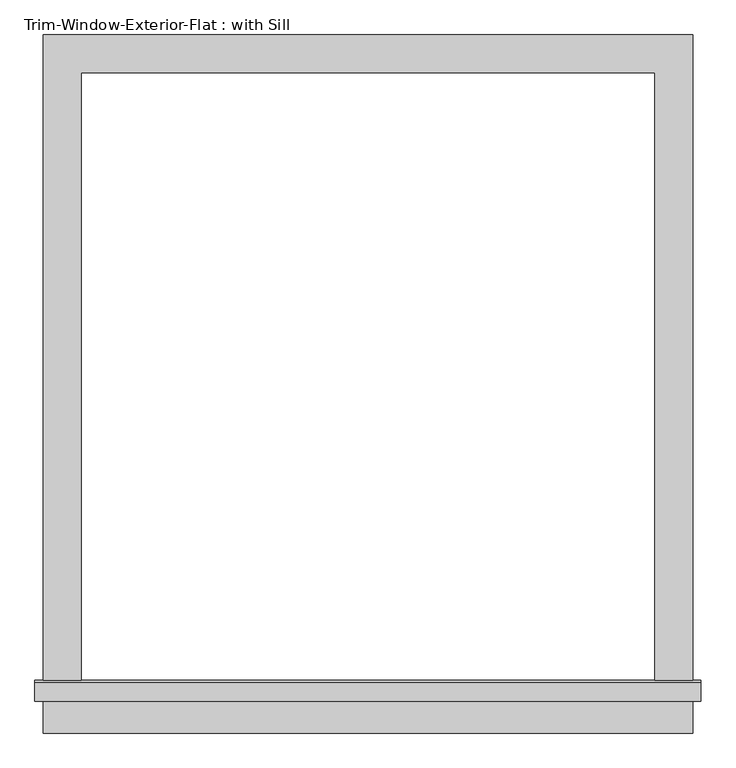
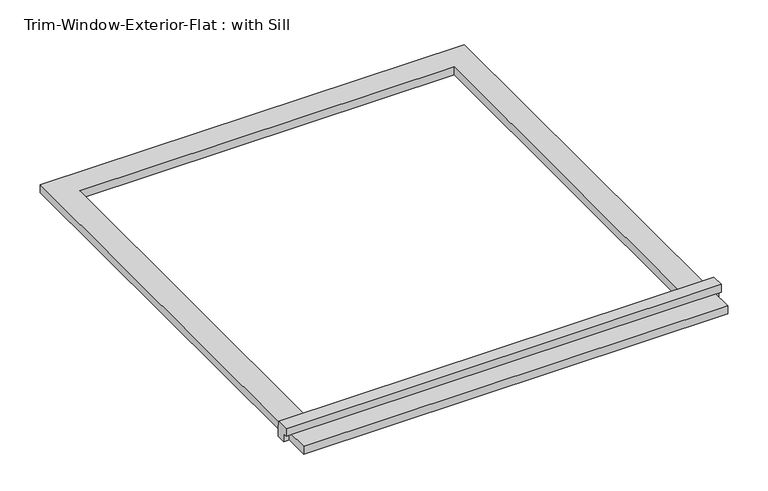
"""IFC4 building model written with IfcOpenShell, lengths in millimetres: proxy geometry, Trim-Window-Exterior-Flat : with Sill."""

import ifcopenshell
import ifcopenshell.guid

model = None  # the IFC model being written
_history = None  # IfcOwnerHistory: only IFC2X3 demands one
_inside = {}  # id of a spatial element -> (the spatial element, [elements in it])
_under = {}  # id of a project, library or spatial element -> (it, [spatial elements below it])
_declared = {}  # id of a project -> (the project, [libraries it declares])
_typed = {}  # id of a type object -> (the type object, [elements of that type])
_made_of = {}  # id of a material, layer set ... -> (it, [elements and type objects made of it])


def new_model(schema):
    """Start an empty IFC model of exactly this schema.

    Asked for "IFC4X3", IfcOpenShell would pick the latest addendum, in which some entities
    have other attributes; the version numbers below select the first issue.
    IFC2X3 requires an IfcOwnerHistory on every rooted entity: one is made here for all.
    """
    global model, _history
    if schema == "IFC4X3":
        model = ifcopenshell.file(schema_version=(4, 3, 0, 0))
    else:
        model = ifcopenshell.file(schema=schema)
    _inside.clear()
    _under.clear()
    _declared.clear()
    _typed.clear()
    _made_of.clear()
    _history = None
    if model.schema == "IFC2X3":
        org = make("IfcOrganization", Name="unknown")
        user = make(
            "IfcPersonAndOrganization",
            ThePerson=make("IfcPerson", FamilyName="unknown"),
            TheOrganization=org,
        )
        app = make(
            "IfcApplication",
            ApplicationDeveloper=org,
            Version="unknown",
            ApplicationFullName="unknown",
            ApplicationIdentifier="unknown",
        )
        _history = make(
            "IfcOwnerHistory",
            OwningUser=user,
            OwningApplication=app,
            ChangeAction="ADDED",
            CreationDate=0,
        )
    return model


def make(cls, **values):
    """One entity of the class cls with the attributes given. An attribute that is None is left unset."""
    return model.create_entity(
        cls, **{name: value for name, value in values.items() if value is not None}
    )


def rooted(cls, **values):
    """An entity with a GlobalId (a new one), such as an element, a storey or a relation."""
    return make(cls, GlobalId=ifcopenshell.guid.new(), OwnerHistory=_history, **values)


def si_unit(unit_type, name, prefix=None):
    """IfcSIUnit, for example si_unit("LENGTHUNIT", "METRE", prefix="MILLI")."""
    return make("IfcSIUnit", UnitType=unit_type, Prefix=prefix, Name=name)


def assignment(units):
    """IfcUnitAssignment: the units of a project."""
    return None if units is None else make("IfcUnitAssignment", Units=units)


def point(xyz):
    """IfcCartesianPoint."""
    return None if xyz is None else make("IfcCartesianPoint", Coordinates=xyz)


def direction(xyz):
    """IfcDirection."""
    return None if xyz is None else make("IfcDirection", DirectionRatios=xyz)


def frame(location, z_axis=None, x_axis=None):
    """IfcAxis2Placement3D, a coordinate frame: its origin and axes. An axis left out is left unset."""
    return make(
        "IfcAxis2Placement3D",
        Location=point(location),
        Axis=direction(z_axis),
        RefDirection=direction(x_axis),
    )


def origin():
    """The frame at (0, 0, 0) with its axes left unset."""
    return frame((0.0, 0.0, 0.0))


def origin_with_axes():
    """The frame at (0, 0, 0) with the z axis (0, 0, 1) and the x axis (1, 0, 0) written out."""
    return frame((0.0, 0.0, 0.0), z_axis=(0.0, 0.0, 1.0), x_axis=(1.0, 0.0, 0.0))


def place(relative_to, where):
    """IfcLocalPlacement: puts the frame where relative to a parent placement (None: the world)."""
    return make(
        "IfcLocalPlacement", PlacementRelTo=relative_to, RelativePlacement=where
    )


def context(
    kind, dimensions, precision=None, world=None, true_north=None, identifier=None
):
    """IfcGeometricRepresentationContext, for example the 3D "Model" context."""
    return make(
        "IfcGeometricRepresentationContext",
        ContextIdentifier=identifier,
        ContextType=kind,
        CoordinateSpaceDimension=dimensions,
        Precision=precision,
        WorldCoordinateSystem=world,
        TrueNorth=true_north,
    )


def project(units=None, contexts=None):
    """IfcProject with its units and contexts."""
    return rooted(
        "IfcProject",
        Name="project",
        RepresentationContexts=contexts,
        UnitsInContext=assignment(units),
    )


def spatial(cls, under=None, at=None, **own):
    """A site, building, storey or space (cls), placed at a placement, below another one or the project."""
    s = rooted(cls, ObjectPlacement=at, **own)
    if under is not None:
        _under.setdefault(under.id(), (under, []))[1].append(s)
    return s


def polyline(points):
    """IfcPolyline through the points."""
    return make("IfcPolyline", Points=[point(p) for p in points])


def outline(outer, holes=None, kind="AREA"):
    """IfcArbitraryClosedProfileDef: a profile drawn as a closed curve; with holes, ...WithVoids."""
    if holes is None:
        return make("IfcArbitraryClosedProfileDef", ProfileType=kind, OuterCurve=outer)
    return make(
        "IfcArbitraryProfileDefWithVoids",
        ProfileType=kind,
        OuterCurve=outer,
        InnerCurves=holes,
    )


def extrude(swept, where, along, depth):
    """IfcExtrudedAreaSolid: the profile swept, set in the frame where, extruded along a direction by depth."""
    return make(
        "IfcExtrudedAreaSolid",
        SweptArea=swept,
        Position=where,
        ExtrudedDirection=direction(along),
        Depth=depth,
    )


def shape(context_of_items, identifier, shape_type, items):
    """IfcShapeRepresentation: the items that make up one representation, for example the "Body"."""
    return make(
        "IfcShapeRepresentation",
        ContextOfItems=context_of_items,
        RepresentationIdentifier=identifier,
        RepresentationType=shape_type,
        Items=items,
    )


def source(mapping_origin, context_of_items, identifier, shape_type, items):
    """IfcRepresentationMap: a shape defined once, which mapped items show again and again."""
    return make(
        "IfcRepresentationMap",
        MappingOrigin=mapping_origin,
        MappedRepresentation=shape(context_of_items, identifier, shape_type, items),
    )


def transform(
    local_origin,
    x_axis=None,
    y_axis=None,
    z_axis=None,
    scale=None,
    scale2=None,
    scale3=None,
    uniform=True,
):
    """IfcCartesianTransformationOperator3D, or its non-uniform kind. x_axis, y_axis, z_axis: its Axis1, 2, 3."""
    if uniform:
        return make(
            "IfcCartesianTransformationOperator3D",
            Axis1=direction(x_axis),
            Axis2=direction(y_axis),
            LocalOrigin=point(local_origin),
            Scale=scale,
            Axis3=direction(z_axis),
        )
    return make(
        "IfcCartesianTransformationOperator3DnonUniform",
        Axis1=direction(x_axis),
        Axis2=direction(y_axis),
        LocalOrigin=point(local_origin),
        Scale=scale,
        Axis3=direction(z_axis),
        Scale2=scale2,
        Scale3=scale3,
    )


def mapped(mapping_source, mapping_target):
    """IfcMappedItem: shows the shape of a source again, moved by a transform."""
    return make(
        "IfcMappedItem", MappingSource=mapping_source, MappingTarget=mapping_target
    )


def made_of(thing, what):
    """Note that an element or type object is made of a material, layer set ...; save() writes the relation."""
    if what is not None:
        _made_of.setdefault(what.id(), (what, []))[1].append(thing)
    return thing


def element(
    cls,
    number,
    at=None,
    inside=None,
    cuts=None,
    type_object=None,
    material=None,
    context=None,
    identifier="Body",
    shape_type=None,
    held_by="IfcProductDefinitionShape",
    body=None,
    shapes=None,
    **own,
):
    """One element of the class cls, such as IfcWall. Its Tag is "e" and its number.

    at: its placement. inside: the storey or other place that contains it. cuts: it is an
    opening in that element (IfcRelVoidsElement). A single representation is given by context,
    identifier, shape_type and body (its items); several are given by shapes. held_by: the class
    of the entity that holds the representations. save() writes the other relations.
    """
    e = rooted(cls, Tag="e%d" % number, ObjectPlacement=at, **own)
    if body is not None:
        shapes = [shape(context, identifier, shape_type, body)]
    if shapes is not None:
        e.Representation = make(held_by, Representations=shapes)
    if inside is not None:
        _inside.setdefault(inside.id(), (inside, []))[1].append(e)
    if cuts is not None:
        rooted(
            "IfcRelVoidsElement", RelatingBuildingElement=cuts, RelatedOpeningElement=e
        )
    if type_object is not None:
        _typed.setdefault(type_object.id(), (type_object, []))[1].append(e)
    return made_of(e, material)


def aggregate(whole, parts):
    """IfcRelAggregates: a whole, such as a stair, and the parts it consists of."""
    return rooted("IfcRelAggregates", RelatingObject=whole, RelatedObjects=parts)


def save(model, path):
    """Write the relations noted so far, then the file.

    IfcRelAggregates (storeys below a building ...), IfcRelContainedInSpatialStructure (elements
    in a storey), IfcRelDefinesByType, IfcRelAssociatesMaterial and IfcRelDeclares: one each for
    every whole, place, type object, material and project.
    """
    for whole, parts in _under.values():
        aggregate(whole, parts)
    for where, things in _inside.values():
        rooted(
            "IfcRelContainedInSpatialStructure",
            RelatedElements=things,
            RelatingStructure=where,
        )
    for kind, things in _typed.values():
        rooted("IfcRelDefinesByType", RelatedObjects=things, RelatingType=kind)
    for what, things in _made_of.values():
        rooted("IfcRelAssociatesMaterial", RelatedObjects=things, RelatingMaterial=what)
    for by, libraries in _declared.values():
        rooted("IfcRelDeclares", RelatingContext=by, RelatedDefinitions=libraries)
    model.write(path)


def trim_window_exterior_flat_with_sill_41619996(model_context):
    return source(origin(), model_context, "Body", "SweptSolid", [
        extrude(outline(polyline([(488.95, -936.5823709), (488.95, -993.7323709), (-488.95, -993.7323709), (-488.95, -936.5823709), (488.95, -936.5823709)])), origin_with_axes(), (0.0, 0.0, 1.0), 19.05),
        extrude(outline(polyline([(-946.15, 38.1), (-916.8580645, 38.1), (-914.4, 19.05), (-914.4, 0.0), (-936.5823709, 0.0), (-936.5823709, 19.05), (-946.15, 19.05), (-946.15, 38.1)])), frame((-501.65, 0.0, 0.0), z_axis=(1.0, 0.0, 0.0), x_axis=(0.0, 1.0, 0.0)), (0.0, 0.0, 1.0), 1003.3),
        extrude(outline(polyline([(-488.95, 57.15), (488.95, 57.15), (488.95, -914.4), (431.8, -914.4), (431.8, 0.0), (-431.8, 0.0), (-431.8, -914.4), (-488.95, -914.4), (-488.95, 57.15)])), origin_with_axes(), (0.0, 0.0, 1.0), 19.05),
    ])


if __name__ == "__main__":
    model = new_model("IFC4")
    model_context = context("Model", 3, world=origin())
    ifc_project = project(units=[si_unit("LENGTHUNIT", "METRE", prefix="MILLI")], contexts=[model_context])
    site = spatial("IfcSite", under=ifc_project)
    building = spatial("IfcBuilding", under=site)
    placement = place(None, origin())
    trim_window_exterior_flat_with_sill_shape = trim_window_exterior_flat_with_sill_41619996(model_context)
    element("IfcBuildingElementProxy", 1, Name="Trim-Window-Exterior-Flat : with Sill", ObjectType="Trim-Window-Exterior-Flat : with Sill", at=placement, inside=building, context=model_context, shape_type="MappedRepresentation", body=[
        mapped(trim_window_exterior_flat_with_sill_shape, transform((0.0, 0.0, 0.0), x_axis=(1.0, 0.0, 0.0), y_axis=(0.0, 1.0, 0.0), z_axis=(0.0, 0.0, 1.0))),
    ])
    save(model, "model.ifc")

# Revit data of these elements
# Type "Trim-Window-Exterior-Flat : with Sill"
#   Trim Width = 0' - 2 1/4"
#   Trim Thickness_Picture Frame = 0' - 1 1/4"
#   Trim Thickness_with Sill = 0' - 0 3/4"
#   Sill Thickness = 0' - 1 1/4"
#   Opening Width [instance default] = 2' - 0"
#   Opening Height [instance default] = 3' - 0"
#   Default Elevation = 4' - 0"
#   Sill = yes
#   Picture Frame = no
#   Trim Material [instance default] = none
# Element 1 (IfcBuildingElementProxy, "Trim-Window-Exterior-Flat : with Sill")
#   Opening Width = 2' - 10"
#   Trim Material = Clad - White
#   Materials on its faces: "Clad - White"
# Materials
#   "Clad - White": class "Wood", colour RGB 216 216 204, transparency 0, Cost = 0
